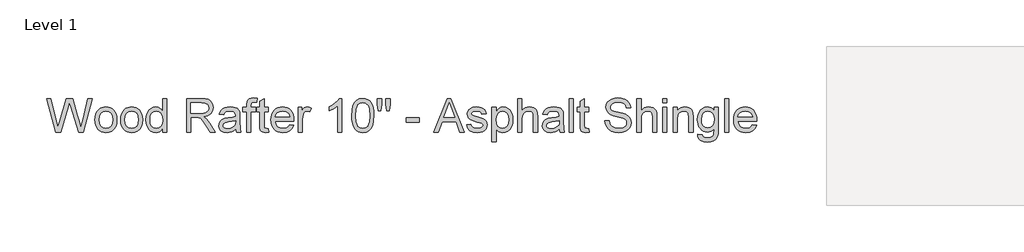
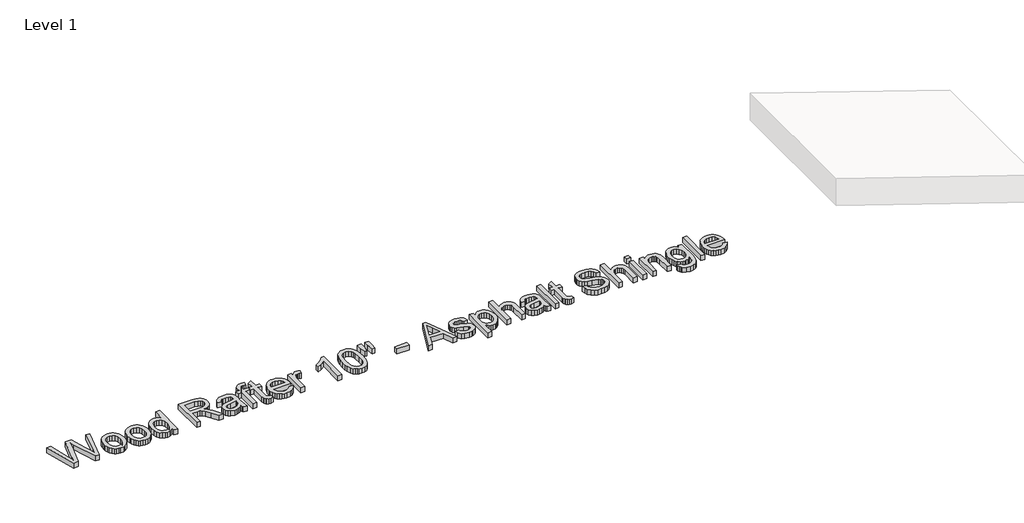
# One storey, part 6 of 42: 1 proxy.
"""IFC4 building model written with IfcOpenShell, lengths in millimetres."""

from ifc_helpers import new_model, si_unit, origin, origin_with_axes, place, context, project, spatial, polyline, outline, extrude, element, save

model = new_model("IFC4")

# Units and contexts
model_context = context("Model", 3, world=origin())
ifc_project = project(units=[si_unit("LENGTHUNIT", "METRE", prefix="MILLI")], contexts=[model_context])

# Site, building, storey
site = spatial("IfcSite", under=ifc_project)
building = spatial("IfcBuilding", under=site)
storey = spatial("IfcBuildingStorey", under=building, Name="Level 1", Elevation=0.0)

# Proxy
placement = place(None, origin())
element("IfcBuildingElementProxy", 1, Name="8\" Arial", ObjectType="8\" Arial", at=placement, inside=storey, context=model_context, shape_type="SweptSolid", body=[
    extrude(outline(polyline([(-8373.4674124, -11588.0070077), (-8456.5244056, -11283.4399136), (-8417.2638036, -11283.4399136), (-8369.0803375, -11483.6094979), (-8354.2088974, -11545.4003317), (-8338.2964564, -11490.7477892), (-8277.9184095, -11283.4399136), (-8221.3325797, -11283.4399136), (-8177.4618313, -11433.7158162), (-8158.6680488, -11489.4837168), (-8144.8190202, -11545.4003317), (-8130.3937233, -11485.3940707), (-8081.764114, -11283.4399136), (-8042.5035121, -11283.4399136), (-8125.6348624, -11588.0070077), (-8166.3082512, -11588.0070077), (-8239.3270223, -11353.0382535), (-8249.5139588, -11320.246728), (-8260.9649677, -11359.7304015), (-8327.5146623, -11588.0070077), (-8373.4674124, -11588.0070077)])), origin_with_axes(), (0.0, 0.0, 1.0), 50.8),
    extrude(outline(polyline([(-8018.7092078, -11476.1737778), (-8016.6504428, -11447.2070008), (-8010.4741479, -11422.246218), (-8000.1803229, -11401.2914294), (-7985.7689679, -11384.342635), (-7971.2600191, -11373.5097203), (-7955.245337, -11365.7719241), (-7937.7249216, -11361.1292464), (-7918.6987729, -11359.5816871), (-7897.6951874, -11361.4661774), (-7878.7038936, -11367.1196483), (-7861.7248915, -11376.5420999), (-7846.7581812, -11389.733532), (-7834.5426873, -11406.2478016), (-7825.8173346, -11425.6387653), (-7820.5821229, -11447.9064232), (-7818.8370523, -11473.0507754), (-7821.9228762, -11511.5120375), (-7831.1803477, -11540.7901852), (-7846.339922, -11562.7162648), (-7867.1320542, -11579.1213222), (-7891.8279395, -11589.3547319), (-7918.6987729, -11592.7658685), (-7940.0090819, -11590.8883492), (-7959.176974, -11585.2557913), (-7976.2024493, -11575.8681947), (-7991.0855078, -11562.7255594), (-8003.1708765, -11546.0509572), (-8011.8032828, -11526.0674595), (-8016.9827266, -11502.7750664), (-8018.7092078, -11476.1737778)]), holes=[polyline([(-7980.6383211, -11476.0994206), (-7976.2326569, -11510.5546885), (-7963.0156645, -11535.1018594), (-7943.1251133, -11549.7967012), (-7918.6987729, -11554.6949818), (-7894.3839683, -11549.7688172), (-7874.5305957, -11534.9903236), (-7861.3136032, -11510.1178399), (-7856.9079391, -11474.9097054), (-7861.3414872, -11441.4582597), (-7874.6421315, -11417.2456963), (-7894.523388, -11402.5508545), (-7918.6987729, -11397.6525739), (-7943.1251133, -11402.5322652), (-7963.0156645, -11417.1713391), (-7976.2326569, -11441.662742), (-7980.6383211, -11476.0994206)])]), origin_with_axes(), (0.0, 0.0, 1.0), 50.8),
    extrude(outline(polyline([(-7785.5250264, -11476.1737778), (-7783.4662614, -11447.2070008), (-7777.2899665, -11422.246218), (-7766.9961415, -11401.2914294), (-7752.5847865, -11384.342635), (-7738.0758377, -11373.5097203), (-7722.0611556, -11365.7719241), (-7704.5407402, -11361.1292464), (-7685.5145915, -11359.5816871), (-7664.511006, -11361.4661774), (-7645.5197122, -11367.1196483), (-7628.5407101, -11376.5420999), (-7613.5739998, -11389.733532), (-7601.3585059, -11406.2478016), (-7592.6331532, -11425.6387653), (-7587.3979415, -11447.9064232), (-7585.652871, -11473.0507754), (-7588.7386948, -11511.5120375), (-7597.9961663, -11540.7901852), (-7613.1557406, -11562.7162648), (-7633.9478728, -11579.1213222), (-7658.6437581, -11589.3547319), (-7685.5145915, -11592.7658685), (-7706.8249005, -11590.8883492), (-7725.9927926, -11585.2557913), (-7743.0182679, -11575.8681947), (-7757.9013264, -11562.7255594), (-7769.9866952, -11546.0509572), (-7778.6191014, -11526.0674595), (-7783.7985452, -11502.7750664), (-7785.5250264, -11476.1737778)]), holes=[polyline([(-7747.4541397, -11476.0994206), (-7743.0484755, -11510.5546885), (-7729.8314831, -11535.1018594), (-7709.9409319, -11549.7967012), (-7685.5145915, -11554.6949818), (-7661.1997869, -11549.7688172), (-7641.3464143, -11534.9903236), (-7628.1294219, -11510.1178399), (-7623.7237577, -11474.9097054), (-7628.1573058, -11441.4582597), (-7641.4579501, -11417.2456963), (-7661.3392066, -11402.5508545), (-7685.5145915, -11397.6525739), (-7709.9409319, -11402.5322652), (-7729.8314831, -11417.1713391), (-7743.0484755, -11441.662742), (-7747.4541397, -11476.0994206)])]), origin_with_axes(), (0.0, 0.0, 1.0), 50.8),
    extrude(outline(polyline([(-7404.8161588, -11588.0070077), (-7404.8161588, -11552.0924797), (-7416.2067525, -11569.8870873), (-7430.0046606, -11582.5975213), (-7446.209883, -11590.2237817), (-7464.8224198, -11592.7658685), (-7489.4346532, -11589.0851871), (-7511.9648851, -11578.0431428), (-7531.037507, -11560.4111916), (-7545.276911, -11536.9607894), (-7554.1440072, -11508.6399906), (-7557.0997059, -11476.3968494), (-7554.3763734, -11444.5533782), (-7546.206376, -11415.7957309), (-7532.5990083, -11391.7597657), (-7513.5635649, -11374.0813413), (-7490.5407166, -11363.2066007), (-7464.9711342, -11359.5816871), (-7446.3446554, -11362.1748945), (-7429.8745355, -11369.9545166), (-7415.9139711, -11381.8795527), (-7404.8161588, -11396.9090019), (-7404.8161588, -11283.4399136), (-7366.7452721, -11283.4399136), (-7366.7452721, -11588.0070077), (-7404.8161588, -11588.0070077)]), holes=[polyline([(-7519.0288191, -11476.248135), (-7514.7346908, -11510.6848136), (-7501.8523058, -11535.1762166), (-7483.1328805, -11549.8152905), (-7461.3276314, -11554.6949818), (-7439.5316769, -11550.0383621), (-7421.2862788, -11536.068503), (-7408.9336888, -11512.5251543), (-7404.8161588, -11479.1480659), (-7409.008046, -11442.6572696), (-7421.5837076, -11417.3572321), (-7440.2938382, -11402.5787384), (-7462.8891326, -11397.6525739), (-7484.9174533, -11402.3835508), (-7502.9676638, -11416.5764815), (-7515.0135303, -11440.9563486), (-7519.0288191, -11476.248135)])]), origin_with_axes(), (0.0, 0.0, 1.0), 50.8),
    extrude(outline(polyline([(-7185.90856, -11588.0070077), (-7185.90856, -11283.4399136), (-7054.6681008, -11283.4399136), (-7019.3949037, -11285.4940313), (-6993.7323748, -11291.6563843), (-6974.9757709, -11303.033036), (-6960.4203489, -11320.7300498), (-6951.0792255, -11342.6747186), (-6947.9655177, -11366.7943356), (-6953.1240485, -11396.7974661), (-6968.5996409, -11421.6699497), (-6980.3225184, -11431.8057656), (-6994.8570274, -11439.9060532), (-7032.3609405, -11450.0000432), (-7010.7229951, -11466.2842701), (-6979.8647568, -11505.4705149), (-6929.0787888, -11588.0070077), (-6973.3213232, -11588.0070077), (-7012.9537112, -11524.8777443), (-7041.5812334, -11483.0889975), (-7061.6948562, -11463.3471607), (-7079.8008346, -11456.0973336), (-7101.8849232, -11454.758904), (-7147.8376732, -11454.758904), (-7147.8376732, -11588.0070077), (-7185.90856, -11588.0070077)]), holes=[polyline([(-7147.8376732, -11416.6880173), (-7062.6243212, -11416.6880173), (-7038.1515075, -11415.340293), (-7019.1625374, -11411.2971202), (-7004.8673656, -11404.288954), (-6994.4759468, -11394.0462497), (-6988.1462901, -11381.6564811), (-6986.0364045, -11368.2071224), (-6990.060988, -11349.6364115), (-7002.1347385, -11334.6720249), (-7022.9082814, -11324.8011065), (-7053.0322423, -11321.5108004), (-7147.8376732, -11321.5108004), (-7147.8376732, -11416.6880173)])]), origin_with_axes(), (0.0, 0.0, 1.0), 50.8),
    extrude(outline(polyline([(-6743.3345014, -11559.4538426), (-6761.5241316, -11575.0502655), (-6780.2528516, -11585.2557913), (-6799.9482151, -11590.8883492), (-6821.0377762, -11592.7658685), (-6852.8533634, -11588.2486686), (-6876.3223549, -11574.6970688), (-6890.7941251, -11554.1187135), (-6895.6180485, -11528.5212471), (-6893.796297, -11512.7389313), (-6888.3310428, -11498.4065808), (-6879.9007952, -11486.1376427), (-6869.1840636, -11476.5455638), (-6842.5270072, -11464.0535541), (-6809.5867672, -11458.3280497), (-6770.6607727, -11452.3051164), (-6743.557573, -11445.2411823), (-6743.3345014, -11436.7644615), (-6745.9555927, -11419.7738411), (-6753.8188667, -11408.6574396), (-6771.4043447, -11400.4037903), (-6795.9050423, -11397.6525739), (-6818.5839885, -11399.48362), (-6834.4220723, -11404.9767582), (-6845.2224557, -11415.1358107), (-6852.7883009, -11430.9645998), (-6890.8591876, -11426.205739), (-6884.2506914, -11405.3857228), (-6874.3890677, -11389.0271386), (-6860.354146, -11376.5165396), (-6841.2257561, -11367.2404788), (-6817.8311219, -11361.496385), (-6790.9974671, -11359.5816871), (-6765.260581, -11361.2733134), (-6744.858824, -11366.3481924), (-6729.4761781, -11373.9791001), (-6718.7966252, -11383.3388128), (-6711.7141018, -11394.9106521), (-6707.1225447, -11409.17794), (-6705.2636147, -11442.4899659), (-6705.2636147, -11489.8555028), (-6703.3303274, -11555.9962328), (-6695.745893, -11588.0070077), (-6733.8167797, -11588.0070077), (-6739.9140702, -11574.771426), (-6743.3345014, -11559.4538426)]), holes=[polyline([(-6743.3345014, -11483.3120691), (-6804.7535492, -11494.9861496), (-6837.5078961, -11501.1577973), (-6852.3421576, -11511.1960194), (-6857.5471617, -11525.8443879), (-6854.7122934, -11537.1652717), (-6846.2076886, -11546.4413325), (-6832.2192402, -11552.6315694), (-6812.9328413, -11554.6949818), (-6792.4846111, -11552.4177925), (-6774.4158113, -11545.5862247), (-6759.7674428, -11535.5201186), (-6749.5805063, -11523.5393147), (-6745.0633063, -11511.1960194), (-6743.557573, -11494.0938632), (-6743.3345014, -11483.3120691)])]), origin_with_axes(), (0.0, 0.0, 1.0), 50.8),
    extrude(outline(polyline([(-6643.3984237, -11588.0070077), (-6643.3984237, -11402.4114347), (-6676.7104496, -11402.4114347), (-6676.7104496, -11364.340548), (-6643.3984237, -11364.340548), (-6643.3984237, -11341.8103162), (-6639.3831348, -11310.0597915), (-6631.7243432, -11297.400478), (-6619.9015483, -11287.3808452), (-6603.3570711, -11280.8560009), (-6581.5332327, -11278.6810528), (-6546.80842, -11282.845056), (-6552.38521, -11318.5365123), (-6574.3205842, -11316.7519395), (-6588.7923544, -11318.33203), (-6598.3007815, -11323.0723016), (-6603.5708481, -11332.1252908), (-6605.3275369, -11346.6435342), (-6605.3275369, -11364.340548), (-6562.4977893, -11364.340548), (-6562.4977893, -11402.4114347), (-6605.3275369, -11402.4114347), (-6605.3275369, -11588.0070077), (-6643.3984237, -11588.0070077)])), origin_with_axes(), (0.0, 0.0, 1.0), 50.8),
    extrude(outline(polyline([(-6448.285129, -11556.256483), (-6443.5262682, -11589.1223657), (-6472.0050761, -11592.7658685), (-6490.2783581, -11591.185778), (-6503.9043152, -11586.4455065), (-6513.5335727, -11579.1399115), (-6519.8167561, -11569.8638507), (-6523.2743659, -11553.9328205), (-6524.4269026, -11526.6623171), (-6524.4269026, -11402.4114347), (-6552.9800676, -11402.4114347), (-6552.9800676, -11364.340548), (-6524.4269026, -11364.340548), (-6524.4269026, -11309.9854343), (-6486.3560158, -11287.6039168), (-6486.3560158, -11364.340548), (-6448.285129, -11364.340548), (-6448.285129, -11402.4114347), (-6486.3560158, -11402.4114347), (-6486.3560158, -11525.5469591), (-6484.3483714, -11545.1772601), (-6477.8421163, -11552.1296583), (-6464.8667848, -11554.6949818), (-6448.285129, -11556.256483)])), origin_with_axes(), (0.0, 0.0, 1.0), 50.8),
    extrude(outline(polyline([(-6253.6179776, -11521.3829559), (-6216.2906629, -11526.1418167), (-6229.7400215, -11554.2674279), (-6251.2013686, -11575.2919264), (-6280.1913822, -11588.397383), (-6316.2267406, -11592.7658685), (-6339.8490938, -11590.8813782), (-6360.8968289, -11585.2279073), (-6379.369946, -11575.8054558), (-6395.2684449, -11562.6140236), (-6408.0532361, -11546.0207496), (-6417.1852298, -11526.3927722), (-6422.6644261, -11503.7300917), (-6424.4908248, -11478.0327078), (-6422.6458368, -11451.4639506), (-6417.1108726, -11428.0460797), (-6407.8859324, -11407.7790952), (-6394.9710161, -11390.662997), (-6379.1143431, -11377.0649239), (-6361.0641326, -11367.3520146), (-6340.8203847, -11361.524269), (-6318.3830994, -11359.5816871), (-6296.6684732, -11361.5196217), (-6277.0312012, -11367.3334253), (-6259.4712835, -11377.023098), (-6243.9887201, -11390.5886398), (-6231.3503197, -11407.6675594), (-6222.3228908, -11427.8973653), (-6216.9064334, -11451.2780576), (-6215.1009476, -11477.8096362), (-6215.3240192, -11488.0709299), (-6386.4199381, -11488.0709299), (-6379.8300311, -11516.5683271), (-6364.5217425, -11537.5184684), (-6342.4283592, -11550.4008534), (-6315.4831686, -11554.6949818), (-6295.2208314, -11552.7059266), (-6278.1558538, -11546.7387613), (-6264.2882359, -11536.4216997), (-6253.6179776, -11521.3829559)]), holes=[polyline([(-6386.4199381, -11450.0000432), (-6253.1718344, -11450.0000432), (-6258.3210706, -11429.8864204), (-6268.4150605, -11415.4983021), (-6290.610685, -11402.1140059), (-6318.5318138, -11397.6525739), (-6344.1943427, -11401.2124249), (-6365.4140289, -11411.8919778), (-6380.1646386, -11428.5386961), (-6386.4199381, -11450.0000432)])]), origin_with_axes(), (0.0, 0.0, 1.0), 50.8),
    extrude(outline(polyline([(-6177.0300609, -11588.0070077), (-6177.0300609, -11364.340548), (-6143.718035, -11364.340548), (-6143.718035, -11397.4295023), (-6131.4119183, -11378.2453445), (-6120.0724452, -11366.94305), (-6108.6957934, -11361.4220278), (-6096.2781409, -11359.5816871), (-6077.3170547, -11362.5187966), (-6058.0585398, -11371.3301248), (-6070.7736211, -11405.46008), (-6084.1579172, -11399.6044504), (-6097.5422133, -11397.6525739), (-6108.9095704, -11399.5300932), (-6119.0686229, -11405.1626512), (-6127.275799, -11414.1226938), (-6132.7875265, -11425.9826674), (-6137.4162622, -11447.2488268), (-6138.9591741, -11470.4482734), (-6138.9591741, -11588.0070077), (-6177.0300609, -11588.0070077)])), origin_with_axes(), (0.0, 0.0, 1.0), 50.8),
    extrude(outline(polyline([(-5782.0446108, -11588.0070077), (-5820.1154975, -11588.0070077), (-5820.1154975, -11350.658823), (-5856.1787399, -11376.3492359), (-5896.257271, -11395.5705723), (-5896.257271, -11359.5816871), (-5866.3563817, -11343.3160495), (-5840.4521919, -11323.964588), (-5820.0318457, -11303.3862327), (-5806.582487, -11283.4399136), (-5782.0446108, -11283.4399136), (-5782.0446108, -11588.0070077)])), origin_with_axes(), (0.0, 0.0, 1.0), 50.8),
    extrude(outline(polyline([(-5691.6262547, -11438.1772483), (-5688.828565, -11389.4268086), (-5680.435496, -11350.5472872), (-5666.5306995, -11320.9438267), (-5647.1978273, -11300.0215694), (-5622.2974597, -11287.5853275), (-5591.690177, -11283.4399136), (-5568.2304802, -11285.8937012), (-5547.224571, -11293.2550641), (-5529.6576823, -11305.2358681), (-5516.5150471, -11321.547979), (-5506.5883608, -11342.0519771), (-5498.6693189, -11366.6084426), (-5493.4829041, -11397.7919936), (-5491.7540992, -11438.1772483), (-5494.523905, -11486.6488485), (-5502.8333221, -11525.4354233), (-5516.6544668, -11555.0667678), (-5535.959455, -11576.072677), (-5560.9155905, -11588.5925706), (-5591.690177, -11592.7658685), (-5612.6589076, -11590.9534118), (-5631.2482077, -11585.5160415), (-5647.4580775, -11576.4537576), (-5661.2885168, -11563.7665602), (-5674.5612772, -11540.8320112), (-5684.0418202, -11512.2556095), (-5689.7301461, -11478.0373552), (-5691.6262547, -11438.1772483)]), holes=[polyline([(-5653.555368, -11438.1028911), (-5649.0939359, -11497.9883216), (-5643.5171459, -11518.4714067), (-5635.7096398, -11532.6480718), (-5615.78191, -11549.1832543), (-5591.690177, -11554.6949818), (-5567.5984439, -11549.164665), (-5547.6707142, -11532.5737146), (-5539.8632081, -11518.3738129), (-5534.286418, -11497.8953751), (-5529.824986, -11438.1028911), (-5534.1377036, -11379.5651848), (-5539.5286007, -11359.1494859), (-5547.0758566, -11344.6358898), (-5566.9664077, -11327.2920727), (-5592.1363202, -11321.5108004), (-5615.967803, -11326.6042686), (-5635.1147822, -11341.8846734), (-5643.1825385, -11357.6855785), (-5648.9452215, -11378.9889165), (-5653.555368, -11438.1028911)])]), origin_with_axes(), (0.0, 0.0, 1.0), 50.8),
    extrude(outline(polyline([(-5449.1474232, -11392.893713), (-5458.4420733, -11334.0771673), (-5458.4420733, -11283.4399136), (-5420.3711866, -11283.4399136), (-5420.3711866, -11334.0771673), (-5428.699193, -11392.893713), (-5449.1474232, -11392.893713)])), origin_with_axes(), (0.0, 0.0, 1.0), 50.8),
    extrude(outline(polyline([(-5373.2287213, -11392.893713), (-5382.3002998, -11334.0771673), (-5382.3002998, -11283.4399136), (-5344.229413, -11283.4399136), (-5344.229413, -11334.0771673), (-5353.1522771, -11392.893713), (-5373.2287213, -11392.893713)])), origin_with_axes(), (0.0, 0.0, 1.0), 50.8),
    extrude(outline(polyline([(-5196.7047269, -11497.5886516), (-5196.7047269, -11459.5177649), (-5077.7332057, -11459.5177649), (-5077.7332057, -11497.5886516), (-5196.7047269, -11497.5886516)])), origin_with_axes(), (0.0, 0.0, 1.0), 50.8),
    extrude(outline(polyline([(-4946.6414609, -11588.0070077), (-4825.0674378, -11283.4399136), (-4792.6476982, -11283.4399136), (-4671.0736751, -11588.0070077), (-4711.3009207, -11588.0070077), (-4746.1744478, -11492.8297908), (-4871.6150454, -11492.8297908), (-4906.4142153, -11588.0070077), (-4946.6414609, -11588.0070077)]), holes=[polyline([(-4857.6358917, -11454.758904), (-4760.0792443, -11454.758904), (-4787.5170514, -11379.8812029), (-4808.857568, -11321.5108004), (-4827.8186542, -11373.3377693), (-4857.6358917, -11454.758904)])]), origin_with_axes(), (0.0, 0.0, 1.0), 50.8),
    extrude(outline(polyline([(-4649.4357297, -11521.3829559), (-4611.3648429, -11516.624095), (-4605.360499, -11532.908322), (-4593.7421864, -11544.8798313), (-4576.4355479, -11552.2411941), (-4553.3662264, -11554.6949818), (-4530.5757444, -11552.4456764), (-4514.5517676, -11545.6977605), (-4505.0712245, -11535.9197886), (-4501.9110435, -11524.5803155), (-4505.0898138, -11514.8767008), (-4514.6261248, -11507.4781593), (-4553.8123696, -11496.622008), (-4611.1417713, -11477.9955292), (-4625.6507201, -11468.6358166), (-4636.1629694, -11456.246048), (-4642.548394, -11441.6162688), (-4644.6768689, -11425.5365241), (-4642.9666532, -11410.7859145), (-4637.8360064, -11397.1692521), (-4629.7496608, -11385.2256267), (-4619.172349, -11375.4941281), (-4594.9690802, -11364.2290122), (-4562.2147333, -11359.5816871), (-4537.4351961, -11361.4499118), (-4515.8901972, -11367.0545858), (-4498.5649695, -11375.8473248), (-4486.4447458, -11387.2797444), (-4478.4141681, -11402.1976578), (-4473.3578784, -11421.4468781), (-4511.4287652, -11426.205739), (-4516.2340993, -11414.224935), (-4525.7425263, -11405.1998298), (-4540.0469928, -11399.5393879), (-4559.2404453, -11397.6525739), (-4581.1014623, -11399.455736), (-4595.6754736, -11404.8652224), (-4603.873355, -11412.6727284), (-4606.6059821, -11421.6699497), (-4602.0701929, -11432.7491726), (-4587.8679675, -11441.1515363), (-4555.076442, -11449.2564712), (-4499.1970057, -11467.1765565), (-4484.4371013, -11475.7462239), (-4473.2463426, -11487.4760723), (-4466.1917032, -11502.4032804), (-4463.8401568, -11520.5650266), (-4466.6006678, -11539.3402198), (-4474.8822011, -11557.000055), (-4488.3687383, -11572.1596293), (-4506.7442616, -11583.4340398), (-4528.939886, -11590.4329114), (-4553.8867268, -11592.7658685), (-4592.2736317, -11588.2672579), (-4620.287707, -11574.771426), (-4638.988543, -11552.4270871), (-4649.4357297, -11521.3829559)])), origin_with_axes(), (0.0, 0.0, 1.0), 50.8),
    extrude(outline(polyline([(-4421.0104091, -11673.6665029), (-4421.0104091, -11364.340548), (-4382.9395224, -11364.340548), (-4382.9395224, -11401.6678627), (-4370.5218699, -11383.2551609), (-4356.6170733, -11370.103231), (-4340.4072036, -11362.2120731), (-4321.0743314, -11359.5816871), (-4295.3281507, -11363.2623686), (-4272.8165082, -11374.3044129), (-4254.4874582, -11392.0386052), (-4241.2890551, -11415.7957309), (-4233.3142453, -11443.8469848), (-4230.6559754, -11474.4635622), (-4233.6581473, -11507.0227215), (-4242.6646633, -11536.1428602), (-4257.387389, -11560.346129), (-4277.5381904, -11578.1546786), (-4301.0071819, -11589.113071), (-4325.6844779, -11592.7658685), (-4343.186304, -11590.3213755), (-4358.8106108, -11582.9878966), (-4372.1856122, -11571.9179684), (-4382.9395224, -11558.2641274), (-4382.9395224, -11673.6665029), (-4421.0104091, -11673.6665029)]), holes=[polyline([(-4382.9395224, -11477.9583506), (-4378.8219924, -11512.0883058), (-4366.4694024, -11535.9569672), (-4348.2425936, -11550.0104781), (-4326.5024071, -11554.6949818), (-4304.4090238, -11549.8431744), (-4285.7174825, -11535.2877524), (-4272.9745172, -11510.5453938), (-4268.7268621, -11475.132777), (-4272.8722761, -11441.1887149), (-4285.3085179, -11416.9854461), (-4303.5074427, -11402.4857919), (-4324.9409058, -11397.6525739), (-4346.4580208, -11402.7925154), (-4365.3540444, -11418.2123399), (-4378.5431529, -11443.4287256), (-4382.9395224, -11477.9583506)])]), origin_with_axes(), (0.0, 0.0, 1.0), 50.8),
    extrude(outline(polyline([(-4187.8262278, -11588.0070077), (-4187.8262278, -11283.4399136), (-4149.755341, -11283.4399136), (-4149.755341, -11395.4218579), (-4135.7715399, -11379.7417832), (-4120.0682286, -11368.5417298), (-4102.645407, -11361.8216978), (-4083.5030752, -11359.5816871), (-4060.5081109, -11362.0261801), (-4040.7476848, -11369.359659), (-4025.1884405, -11381.0058556), (-4014.7970217, -11396.3885015), (-4008.9413922, -11417.5245358), (-4006.9895157, -11446.4308975), (-4006.9895157, -11588.0070077), (-4045.0604024, -11588.0070077), (-4045.0604024, -11450.3718292), (-4048.0904583, -11426.5403464), (-4057.1806261, -11410.2189408), (-4071.8289947, -11400.7941656), (-4091.5336528, -11397.6525739), (-4107.6226921, -11399.7717541), (-4122.7264985, -11406.1292948), (-4135.2370976, -11416.111749), (-4143.5465147, -11429.1056698), (-4148.2031344, -11446.3751296), (-4149.755341, -11469.184201), (-4149.755341, -11588.0070077), (-4187.8262278, -11588.0070077)])), origin_with_axes(), (0.0, 0.0, 1.0), 50.8),
    extrude(outline(polyline([(-3811.876221, -11559.4538426), (-3830.0658512, -11575.0502655), (-3848.7945712, -11585.2557913), (-3868.4899347, -11590.8883492), (-3889.5794957, -11592.7658685), (-3921.395083, -11588.2486686), (-3944.8640745, -11574.6970688), (-3959.3358447, -11554.1187135), (-3964.159768, -11528.5212471), (-3962.3380166, -11512.7389313), (-3956.8727624, -11498.4065808), (-3948.4425147, -11486.1376427), (-3937.7257832, -11476.5455638), (-3911.0687267, -11464.0535541), (-3878.1284868, -11458.3280497), (-3839.2024923, -11452.3051164), (-3812.0992926, -11445.2411823), (-3811.876221, -11436.7644615), (-3814.4973123, -11419.7738411), (-3822.3605863, -11408.6574396), (-3839.9460643, -11400.4037903), (-3864.4467619, -11397.6525739), (-3887.1257081, -11399.48362), (-3902.9637919, -11404.9767582), (-3913.7641753, -11415.1358107), (-3921.3300204, -11430.9645998), (-3959.4009072, -11426.205739), (-3952.792411, -11405.3857228), (-3942.9307872, -11389.0271386), (-3928.8958656, -11376.5165396), (-3909.7674757, -11367.2404788), (-3886.3728415, -11361.496385), (-3859.5391867, -11359.5816871), (-3833.8023006, -11361.2733134), (-3813.4005436, -11366.3481924), (-3798.0178977, -11373.9791001), (-3787.3383448, -11383.3388128), (-3780.2558214, -11394.9106521), (-3775.6642643, -11409.17794), (-3773.8053343, -11442.4899659), (-3773.8053343, -11489.8555028), (-3771.872047, -11555.9962328), (-3764.2876126, -11588.0070077), (-3802.3584993, -11588.0070077), (-3808.4557898, -11574.771426), (-3811.876221, -11559.4538426)]), holes=[polyline([(-3811.876221, -11483.3120691), (-3873.2952688, -11494.9861496), (-3906.0496157, -11501.1577973), (-3920.8838772, -11511.1960194), (-3926.0888813, -11525.8443879), (-3923.254013, -11537.1652717), (-3914.7494082, -11546.4413325), (-3900.7609598, -11552.6315694), (-3881.4745609, -11554.6949818), (-3861.0263307, -11552.4177925), (-3842.9575309, -11545.5862247), (-3828.3091624, -11535.5201186), (-3818.1222259, -11523.5393147), (-3813.6050259, -11511.1960194), (-3812.0992926, -11494.0938632), (-3811.876221, -11483.3120691)])]), origin_with_axes(), (0.0, 0.0, 1.0), 50.8),
    extrude(outline(polyline([(-3721.457865, -11588.0070077), (-3721.457865, -11283.4399136), (-3683.3869782, -11283.4399136), (-3683.3869782, -11588.0070077), (-3721.457865, -11588.0070077)])), origin_with_axes(), (0.0, 0.0, 1.0), 50.8),
    extrude(outline(polyline([(-3545.3800137, -11556.256483), (-3540.6211529, -11589.1223657), (-3569.0999607, -11592.7658685), (-3587.3732428, -11591.185778), (-3600.9991998, -11586.4455065), (-3610.6284573, -11579.1399115), (-3616.9116408, -11569.8638507), (-3620.3692506, -11553.9328205), (-3621.5217872, -11526.6623171), (-3621.5217872, -11402.4114347), (-3650.0749523, -11402.4114347), (-3650.0749523, -11364.340548), (-3621.5217872, -11364.340548), (-3621.5217872, -11309.9854343), (-3583.4509005, -11287.6039168), (-3583.4509005, -11364.340548), (-3545.3800137, -11364.340548), (-3545.3800137, -11402.4114347), (-3583.4509005, -11402.4114347), (-3583.4509005, -11525.5469591), (-3581.443256, -11545.1772601), (-3574.937001, -11552.1296583), (-3561.9616695, -11554.6949818), (-3545.3800137, -11556.256483)])), origin_with_axes(), (0.0, 0.0, 1.0), 50.8),
    extrude(outline(polyline([(-3397.8553275, -11483.3120691), (-3359.7844408, -11483.3120691), (-3355.4159552, -11504.4388087), (-3347.5155026, -11521.4201345), (-3335.1907966, -11534.8973771), (-3317.5495508, -11545.5118675), (-3295.9859626, -11552.3992032), (-3271.8942295, -11554.6949818), (-3250.683838, -11552.9568822), (-3232.1131272, -11547.7425835), (-3217.0650887, -11539.4889342), (-3206.4227143, -11528.6327829), (-3200.0930576, -11516.1686572), (-3197.983172, -11503.0910845), (-3199.5632625, -11490.3481192), (-3204.3035341, -11479.3339589), (-3213.9327916, -11469.9370676), (-3230.1798399, -11462.0459097), (-3285.6131331, -11447.509077), (-3322.0016881, -11437.8891141), (-3345.2847866, -11428.7338838), (-3364.2365781, -11415.925856), (-3377.6673475, -11400.4037903), (-3385.6700412, -11382.5022942), (-3388.3376058, -11362.5559752), (-3385.038005, -11340.2581096), (-3375.1392027, -11319.4659773), (-3358.901449, -11301.8433208), (-3336.5849941, -11289.0538823), (-3309.7978126, -11281.2742601), (-3280.1478788, -11278.6810528), (-3248.0255681, -11281.3950906), (-3219.9185462, -11289.5372041), (-3196.8306354, -11302.9400895), (-3179.7656579, -11321.4364432), (-3168.9652745, -11343.8737285), (-3164.6711461, -11369.0994088), (-3202.7420329, -11369.0994088), (-3209.7316097, -11346.383284), (-3224.3056211, -11329.9875212), (-3247.0775138, -11320.060835), (-3278.6607348, -11316.7519395), (-3310.9875278, -11320.0236564), (-3333.1645629, -11329.8388068), (-3345.99118, -11344.2826931), (-3350.2667191, -11361.4406171), (-3347.2366631, -11376.0703964), (-3338.1464954, -11387.8374234), (-3316.6572643, -11398.3589673), (-3275.9838756, -11409.1035828), (-3234.0092358, -11419.3091086), (-3208.6162517, -11428.2133834), (-3186.9132438, -11442.0252334), (-3171.7722588, -11459.0716217), (-3162.8772787, -11479.1666552), (-3159.9122853, -11502.1244409), (-3163.3234219, -11525.5934323), (-3173.5568316, -11547.6682263), (-3190.1942553, -11566.6664911), (-3212.8174336, -11580.905895), (-3240.0228744, -11589.8008751), (-3270.4070855, -11592.7658685), (-3307.7065163, -11589.5685089), (-3338.4067456, -11579.97643), (-3362.8609699, -11563.9524533), (-3381.4223862, -11541.4594), (-3393.3381276, -11514.0587716), (-3397.8553275, -11483.3120691)])), origin_with_axes(), (0.0, 0.0, 1.0), 50.8),
    extrude(outline(polyline([(-3107.564816, -11588.0070077), (-3107.564816, -11283.4399136), (-3069.4939292, -11283.4399136), (-3069.4939292, -11395.4218579), (-3055.5101282, -11379.7417832), (-3039.8068168, -11368.5417298), (-3022.3839953, -11361.8216978), (-3003.2416634, -11359.5816871), (-2980.2466991, -11362.0261801), (-2960.486273, -11369.359659), (-2944.9270287, -11381.0058556), (-2934.53561, -11396.3885015), (-2928.6799804, -11417.5245358), (-2926.7281039, -11446.4308975), (-2926.7281039, -11588.0070077), (-2964.7989906, -11588.0070077), (-2964.7989906, -11450.3718292), (-2967.8290466, -11426.5403464), (-2976.9192143, -11410.2189408), (-2991.5675829, -11400.7941656), (-3011.2722411, -11397.6525739), (-3027.3612804, -11399.7717541), (-3042.4650868, -11406.1292948), (-3054.9756858, -11416.111749), (-3063.285103, -11429.1056698), (-3067.9417227, -11446.3751296), (-3069.4939292, -11469.184201), (-3069.4939292, -11588.0070077), (-3107.564816, -11588.0070077)])), origin_with_axes(), (0.0, 0.0, 1.0), 50.8),
    extrude(outline(polyline([(-2874.3806346, -11321.5108004), (-2874.3806346, -11283.4399136), (-2836.3097478, -11283.4399136), (-2836.3097478, -11321.5108004), (-2874.3806346, -11321.5108004)])), origin_with_axes(), (0.0, 0.0, 1.0), 50.8),
    extrude(outline(polyline([(-2874.3806346, -11588.0070077), (-2874.3806346, -11364.340548), (-2836.3097478, -11364.340548), (-2836.3097478, -11588.0070077), (-2874.3806346, -11588.0070077)])), origin_with_axes(), (0.0, 0.0, 1.0), 50.8),
    extrude(outline(polyline([(-2779.2034177, -11588.0070077), (-2779.2034177, -11364.340548), (-2741.1325309, -11364.340548), (-2741.1325309, -11395.5705723), (-2727.9062439, -11379.825435), (-2712.0216869, -11368.5789084), (-2693.4788599, -11361.8309924), (-2672.2777631, -11359.5816871), (-2653.5118646, -11361.3941439), (-2636.3260565, -11366.8315142), (-2621.9937061, -11375.2152886), (-2611.7881803, -11385.8669576), (-2600.37435, -11413.8624436), (-2598.3667056, -11450.669258), (-2598.3667056, -11588.0070077), (-2636.4375923, -11588.0070077), (-2636.4375923, -11455.7999048), (-2640.8246672, -11422.1160929), (-2646.8940737, -11412.0871655), (-2656.3281435, -11404.3075433), (-2668.4204833, -11399.3163163), (-2682.4646996, -11397.6525739), (-2704.7625651, -11401.3890232), (-2723.7701246, -11412.5983712), (-2731.3661773, -11421.7489542), (-2736.7919293, -11434.2549059), (-2741.1325309, -11469.3329154), (-2741.1325309, -11588.0070077), (-2779.2034177, -11588.0070077)])), origin_with_axes(), (0.0, 0.0, 1.0), 50.8),
    extrude(outline(polyline([(-2555.536958, -11607.0424511), (-2517.4660712, -11611.8013119), (-2513.2648894, -11623.698464), (-2505.1227759, -11631.8777561), (-2489.1173885, -11638.2352968), (-2468.1672472, -11640.354477), (-2445.8229083, -11637.9564572), (-2429.204074, -11630.7623981), (-2417.6787079, -11619.237032), (-2410.6147738, -11603.8450914), (-2408.0122718, -11559.4538426), (-2420.6808799, -11571.9458523), (-2434.8180426, -11580.8687164), (-2450.4237601, -11586.2224349), (-2467.4980324, -11588.0070077), (-2488.3714928, -11585.9296534), (-2506.7493397, -11579.6975905), (-2522.631573, -11569.310819), (-2536.0181928, -11554.769339), (-2546.6396542, -11537.3232808), (-2554.2264123, -11518.2227748), (-2558.7784672, -11497.4678212), (-2560.2958188, -11475.0584198), (-2557.5724864, -11444.321012), (-2549.4024889, -11416.0559811), (-2536.0739607, -11392.1036678), (-2517.8750358, -11374.3044129), (-2495.4284559, -11363.2623686), (-2469.3569624, -11359.5816871), (-2451.5530601, -11361.6636887), (-2435.3943109, -11367.9096936), (-2420.8807148, -11378.3197017), (-2408.0122718, -11392.893713), (-2408.0122718, -11364.340548), (-2369.941385, -11364.340548), (-2369.941385, -11557.4461982), (-2372.5438871, -11602.0326347), (-2380.3513931, -11631.3944343), (-2393.8007518, -11650.8667262), (-2413.3288116, -11665.7846396), (-2438.5080187, -11675.2651827), (-2468.9108192, -11678.4253637), (-2504.3327306, -11673.9732263), (-2532.2259756, -11660.6168142), (-2542.7312538, -11650.5902104), (-2550.118177, -11638.3189486), (-2554.386745, -11623.8030288), (-2555.536958, -11607.0424511)]), holes=[polyline([(-2522.2249321, -11472.4559178), (-2518.16317, -11507.3759182), (-2505.9778837, -11531.3839993), (-2487.6581284, -11545.2980905), (-2465.1929591, -11549.9361209), (-2442.8950936, -11545.3259745), (-2424.4823917, -11531.4955351), (-2412.1298018, -11507.7941774), (-2408.0122718, -11473.5712758), (-2412.2506322, -11440.5659733), (-2424.9657136, -11416.7995531), (-2443.6479602, -11402.4393187), (-2465.7878167, -11397.6525739), (-2487.5280033, -11402.3649615), (-2505.7548121, -11416.5021243), (-2518.1074021, -11439.9153478), (-2522.2249321, -11472.4559178)])]), origin_with_axes(), (0.0, 0.0, 1.0), 50.8),
    extrude(outline(polyline([(-2312.8350549, -11588.0070077), (-2312.8350549, -11283.4399136), (-2274.7641681, -11283.4399136), (-2274.7641681, -11588.0070077), (-2312.8350549, -11588.0070077)])), origin_with_axes(), (0.0, 0.0, 1.0), 50.8),
    extrude(outline(polyline([(-2061.0615733, -11521.3829559), (-2023.7342586, -11526.1418167), (-2037.1836172, -11554.2674279), (-2058.6449643, -11575.2919264), (-2087.6349779, -11588.397383), (-2123.6703363, -11592.7658685), (-2147.2926895, -11590.8813782), (-2168.3404246, -11585.2279073), (-2186.8135417, -11575.8054558), (-2202.7120407, -11562.6140236), (-2215.4968319, -11546.0207496), (-2224.6288256, -11526.3927722), (-2230.1080218, -11503.7300917), (-2231.9344205, -11478.0327078), (-2230.0894325, -11451.4639506), (-2224.5544684, -11428.0460797), (-2215.3295282, -11407.7790952), (-2202.4146119, -11390.662997), (-2186.5579388, -11377.0649239), (-2168.5077283, -11367.3520146), (-2148.2639804, -11361.524269), (-2125.8266951, -11359.5816871), (-2104.1120689, -11361.5196217), (-2084.4747969, -11367.3334253), (-2066.9148792, -11377.023098), (-2051.4323158, -11390.5886398), (-2038.7939154, -11407.6675594), (-2029.7664865, -11427.8973653), (-2024.3500291, -11451.2780576), (-2022.5445434, -11477.8096362), (-2022.767615, -11488.0709299), (-2193.8635338, -11488.0709299), (-2187.2736269, -11516.5683271), (-2171.9653382, -11537.5184684), (-2149.8719549, -11550.4008534), (-2122.9267643, -11554.6949818), (-2102.6644271, -11552.7059266), (-2085.5994496, -11546.7387613), (-2071.7318316, -11536.4216997), (-2061.0615733, -11521.3829559)]), holes=[polyline([(-2193.8635338, -11450.0000432), (-2060.6154301, -11450.0000432), (-2065.7646663, -11429.8864204), (-2075.8586563, -11415.4983021), (-2098.0542807, -11402.1140059), (-2125.9754095, -11397.6525739), (-2151.6379384, -11401.2124249), (-2172.8576246, -11411.8919778), (-2187.6082343, -11428.5386961), (-2193.8635338, -11450.0000432)])]), origin_with_axes(), (0.0, 0.0, 1.0), 50.8),
])

save(model, "model.ifc")

# Revit data of these elements
# Element 1 (IfcBuildingElementProxy, "8\" Arial")
#   Phase Created = New Construction
